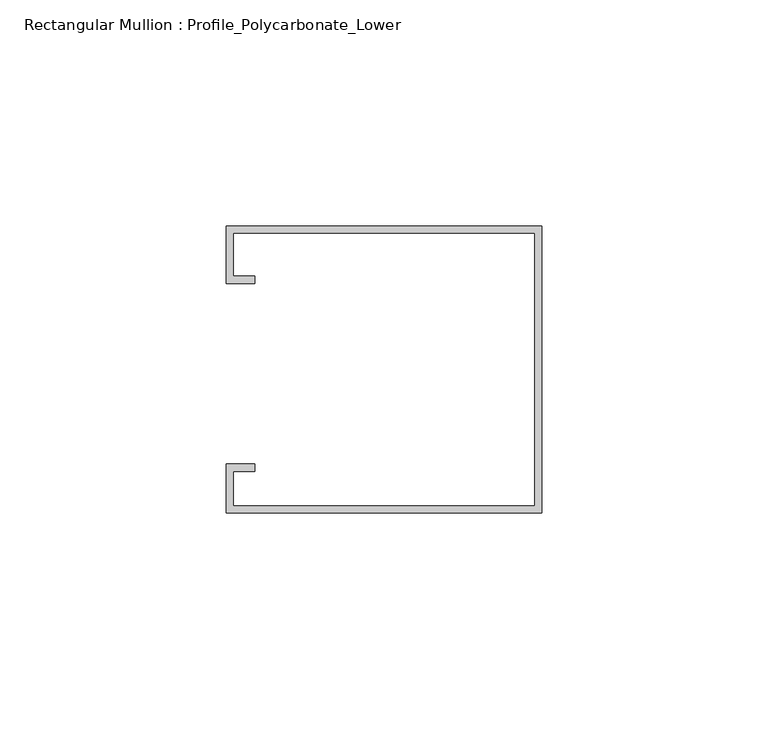
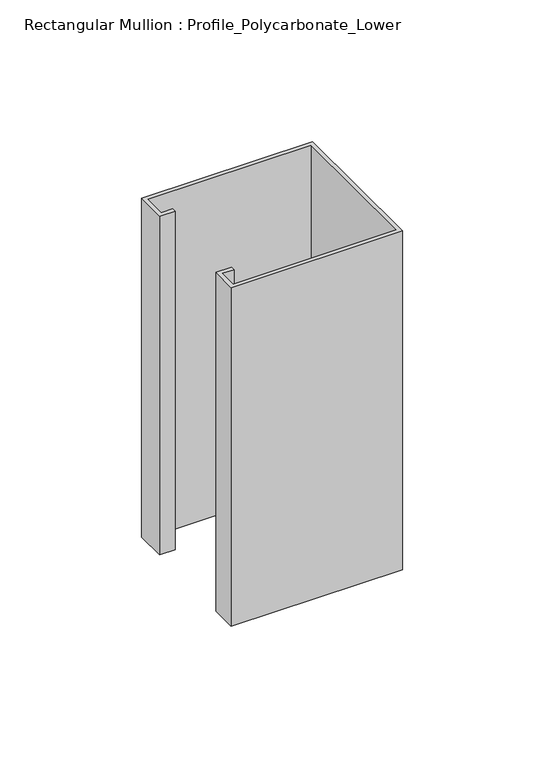
"""IFC4 building model written with IfcOpenShell, lengths in millimetres: member geometry, Rectangular Mullion : Profile_Polycarbonate_Lower."""

from ifc_helpers import new_model, si_unit, frame, origin, place, context, project, spatial, polyline, outline, extrude, source, transform, mapped, element, save


def rectangular_mullion_profile_polycarbonate_lower_8b1fbbc3(model_context):
    return source(origin(), model_context, "Body", "SweptSolid", [
        extrude(outline(polyline([(0.0, 32.7), (0.0, -30.8), (-69.85, -30.8), (-69.85, -20.0), (-63.5, -20.0), (-63.5, -21.5875), (-68.2625, -21.5875), (-68.2625, -29.2125), (-1.5875, -29.2125), (-1.5875, 31.1125), (-68.2625, 31.1125), (-68.2625, 21.5875), (-63.5, 21.5875), (-63.5, 20.0), (-69.85, 20.0), (-69.85, 32.7), (0.0, 32.7)])), frame((0.0, 0.0, -146.05), z_axis=(0.0, 0.0, 1.0), x_axis=(1.0, 0.0, 0.0)), (0.0, 0.0, 1.0), 146.05),
    ])


if __name__ == "__main__":
    model = new_model("IFC4")
    model_context = context("Model", 3, world=origin())
    ifc_project = project(units=[si_unit("LENGTHUNIT", "METRE", prefix="MILLI")], contexts=[model_context])
    site = spatial("IfcSite", under=ifc_project)
    building = spatial("IfcBuilding", under=site)
    placement = place(None, origin())
    rectangular_mullion_profile_polycarbonate_lower_shape = rectangular_mullion_profile_polycarbonate_lower_8b1fbbc3(model_context)
    element("IfcMember", 1, ObjectType="Rectangular Mullion : Profile_Polycarbonate_Lower", at=placement, inside=building, context=model_context, shape_type="MappedRepresentation", body=[
        mapped(rectangular_mullion_profile_polycarbonate_lower_shape, transform((0.0, 0.0, 0.0), x_axis=(1.0, 0.0, 0.0), y_axis=(0.0, 1.0, 0.0), z_axis=(0.0, 0.0, 1.0))),
    ])
    save(model, "model.ifc")

# Revit data of these elements
# Type "Rectangular Mullion : Profile_Polycarbonate_Lower"
#   built-in parameter 1007322 = 0.208333 (stored number, unit not read)
#   built-in parameter 1007321 = 0 (stored number, unit not read)
#   built-in parameter 1007320 = 0.00520833 (stored number, unit not read)
